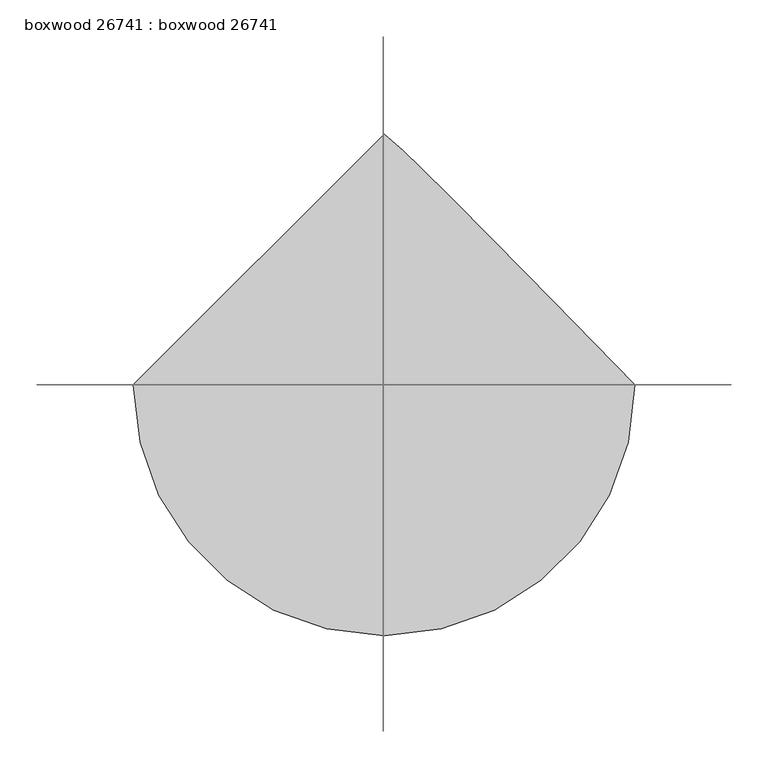
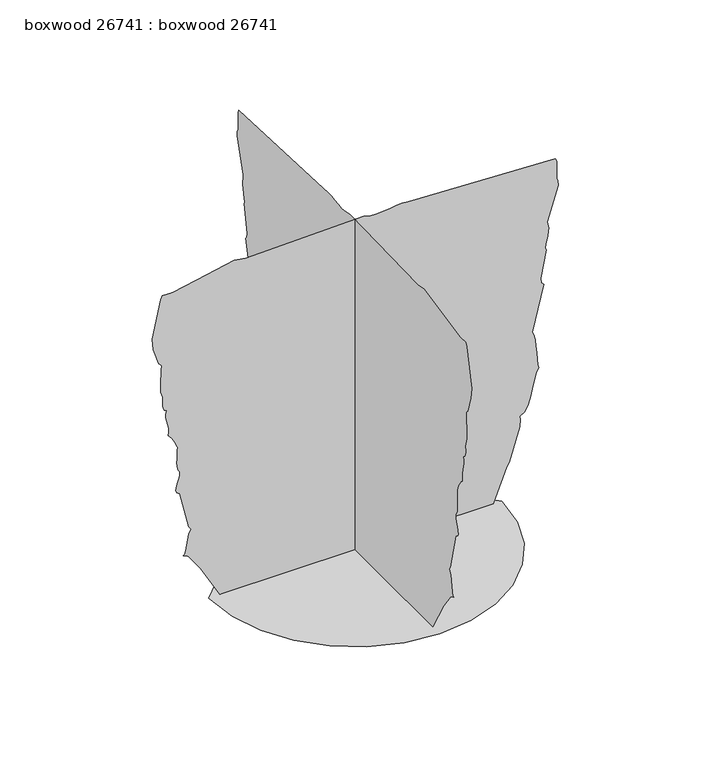
"""IFC4 building model written with IfcOpenShell, lengths in millimetres: proxy geometry, boxwood 26741 : boxwood 26741."""

from ifc_helpers import new_model, si_unit, origin, place, context, project, spatial, triangles, source, transform, mapped, element, save


def boxwood_26741_boxwood_26741_9aa5a226(model_context):
    return source(origin(), model_context, "Body", "Tessellation", [
        triangles([(-340.161904, 0.0, 0.0), (-331.1677583, -77.9424445, 0.0), (-305.5569305, -149.5201522, 0.0), (-265.3792049, -212.6823306, 0.0), (-212.6823306, -265.3792049, 0.0), (-149.5201522, -305.5569305, 0.0), (-77.9424445, -331.1677583, 0.0), (1.49e-05, -340.161904, 0.0), (77.9424445, -331.1677583, 0.0), (149.5201522, -305.5569305, 0.0), (212.6823306, -265.3792049, 0.0), (265.3792049, -212.6823306, 0.0), (305.5569305, -149.5201522, 0.0), (331.1677583, -77.9424445, 0.0), (340.161904, 2.97e-05, 0.0), (229.6165077, 113.3919522, 0.0), (147.6639246, 196.877445, 0.0), (89.5385572, 255.4401858, 0.0), (50.4748806, 294.0659713, 0.0), (25.7075946, 317.7387815, 0.0), (10.4710485, 331.4420875, 0.0), (-4.46e-05, 340.161904, 0.0), (-314.391057, 3.72e-05, 1.1804295), (-359.6030502, 3.25e-05, 80.9365932), (-387.8072153, 3.02e-05, 119.3439327), (-399.7375917, 2.98e-05, 125.1409807), (-396.5295753, 2.97e-05, 127.6759005), (-393.8092472, 2.92e-05, 136.0634881), (-391.3784363, 2.85e-05, 147.9626255), (-389.0442038, 2.77e-05, 161.0321948), (-386.6159363, 2.7e-05, 172.9315956), (-383.8930647, 2.65e-05, 181.3191832), (-380.6875917, 2.64e-05, 183.8540939), (-386.4178379, 2.59e-05, 191.475867), (-407.8706709, 2.06e-05, 279.9816748), (-415.0715758, 2.03e-05, 285.8922515), (-417.4159822, 1.99e-05, 291.1246538), (-416.3669546, 1.95e-05, 298.5846272), (-413.3773842, 1.9e-05, 307.4187355), (-409.9052124, 1.84e-05, 316.7735787), (-407.3982433, 1.79e-05, 325.7905792), (-407.3144185, 1.74e-05, 333.6213876), (-411.0989985, 1.7e-05, 339.4049735), (-412.8821019, 1.68e-05, 343.3826014), (-413.8320439, 1.64e-05, 350.1263031), (-414.1444885, 1.59e-05, 358.7927799), (-414.0123745, 1.54e-05, 368.5362259), (-413.6237718, 1.48e-05, 378.5158856), (-413.1741989, 1.42e-05, 387.8859532), (-412.8516169, 1.37e-05, 395.8056733), (-413.5475773, 1.36e-05, 397.7894185), (-415.5668581, 1.33e-05, 402.5595489), (-418.5996308, 1.29e-05, 409.0720874), (-422.335958, 1.25e-05, 416.2857096), (-426.4660111, 1.21e-05, 423.1538587), (-430.6849397, 1.17e-05, 428.6300869), (-434.6803717, 1.15e-05, 431.6729971), (-433.0471501, 1.1e-05, 440.9821309), (-433.7685087, 1.04e-05, 450.5350362), (-435.8335353, 9.9e-06, 460.1032385), (-438.2363683, 9.3e-06, 469.4580454), (-439.9737259, 8.8e-06, 478.3709098), (-440.034696, 8.3e-06, 486.6106685), (-437.4134171, 7.8e-06, 493.9512815), (-443.2020899, 7.6e-06, 497.9797056), (-446.1205164, 7.3e-06, 503.1613297), (-447.0831757, 6.9e-06, 509.2624108), (-447.0095246, 6.6e-06, 516.0543654), (-446.8114263, 6.1e-06, 523.3111536), (-447.4083012, 5.6e-06, 530.7990686), (-449.7146284, 5.2e-06, 538.2920706), (-451.312278, 4.9e-06, 544.3448625), (-452.0082384, 4.4e-06, 552.960543), (-452.0184122, 3.7e-06, 563.4380648), (-451.5713828, 3e-06, 575.0738008), (-450.8830164, 2.3e-06, 587.161653), (-450.1769185, 1.6e-06, 599.0006106), (-449.6740059, 1e-06, 609.884503), (-455.9351063, 5e-07, 616.20403), (-468.9576762, -1.9e-06, 655.9295849), (-471.3528789, -3.4e-06, 681.38806), (-452.1758881, -8.8e-06, 772.6680262), (-448.2312887, -9.3e-06, 780.8340975), (-424.9242448, -9.2e-06, 779.2695127), (-369.5370006, -9.9e-06, 791.4970367), (-280.9036933, -1.1e-05, 809.3710184), (-254.2463815, -1.07e-05, 804.8396816), (19.1367407, -1.11e-05, 811.6748022), (35.370009, -1.09e-05, 807.659059), (50.7118619, -1.08e-05, 806.6938562), (65.4184633, -1.09e-05, 807.7555647), (79.7468584, -1.1e-05, 809.8129972), (93.9523139, -1.11e-05, 811.837365), (108.2921454, -1.11e-05, 812.8000242), (123.0221057, -1.11e-05, 811.6748022), (464.7514286, -1.02e-05, 797.3212452), (467.4463586, -9.9e-06, 790.6791361), (467.5250965, -7.3e-06, 748.7767519), (470.2200628, -6.9e-06, 742.132172), (471.0074421, -6.3e-06, 730.722476), (446.1992907, -1.4e-06, 649.650753), (447.5784943, -8e-07, 638.6728621), (448.9932698, -4e-07, 632.8486536), (448.3227076, 0.0, 624.6114384), (446.3999325, 6e-07, 614.9264191), (444.0605767, 1.2e-06, 604.756255), (442.1378016, 1.8e-06, 595.0686922), (441.4672394, 2.3e-06, 586.8314406), (442.8795078, 2.7e-06, 581.0072322), (430.5681227, 6.5e-06, 516.2728114), (432.2445102, 7.2e-06, 504.59896), (437.7537669, 7.6e-06, 498.820461), (410.7154827, 1.41e-05, 389.8950966), (414.6016554, 1.45e-05, 382.811045), (417.3397877, 1.52e-05, 370.1135642), (419.2981347, 1.62e-05, 353.9591723), (420.8348505, 1.72e-05, 336.5119088), (422.3156467, 1.82e-05, 319.9231685), (424.1038007, 1.9e-05, 306.3570271), (426.5625169, 1.95e-05, 297.9699481), (420.4843268, 2.02e-05, 287.3705225), (415.6710305, 2.11e-05, 270.9595874), (411.3047636, 2.23e-05, 251.374918), (406.5625749, 2.35e-05, 231.2497293), (400.6266, 2.46e-05, 213.2215782), (392.6738514, 2.54e-05, 199.9259508), (381.8813779, 2.58e-05, 193.9993685), (383.6035111, 2.63e-05, 184.6265031), (381.7493002, 2.73e-05, 168.2889829), (357.4541988, 3.19e-05, 89.6124717), (351.8814649, 3.25e-05, 80.6919951), (319.8571115, 3.72e-05, 1.0471049), (-1.3669569, -313.0245343, 1.1804269), (-1.3669569, -358.2365275, 80.9365932), (-1.3669569, -386.4381492, 119.3439327), (-1.3669569, -398.371069, 125.1409807), (-1.3669569, -395.1630527, 127.6759005), (-1.3669569, -392.4427245, 136.0634881), (-1.3669569, -390.0119136, 147.9626255), (-1.3669569, -387.6776811, 161.0324491), (-1.3669569, -385.2469065, 172.9315956), (-1.3669569, -382.526542, 181.3191832), (-1.3669569, -379.3185256, 183.8540939), (-1.3669569, -385.0513152, 191.475867), (-1.3669569, -406.5041482, 279.9816748), (-1.3669569, -413.7050531, 285.8922515), (-1.3669569, -416.046916, 291.1246538), (-1.3669569, -414.9979248, 298.5846272), (-1.3669569, -412.0108615, 307.4187355), (-1.3669569, -408.5386897, 316.7735787), (-1.3669569, -406.0317206, 325.7905792), (-1.3669569, -405.9453524, 333.6213876), (-1.3669569, -409.7324759, 339.4049735), (-1.3669569, -411.5130358, 343.3826014), (-1.3669569, -412.4655212, 350.1263031), (-1.3669569, -412.7779658, 358.7927799), (-1.3669569, -412.6458881, 368.5362259), (-1.3669569, -412.2572491, 378.5158856), (-1.3669569, -411.8076762, 387.8859532), (-1.3669569, -411.4850942, 395.8056733), (-1.3669569, -412.1810546, 397.7894185), (-1.3669569, -414.2003354, 402.5595489), (-1.3669569, -417.2331081, 409.0720874), (-1.3669569, -420.9669282, 416.2857096), (-1.3669569, -425.0994884, 423.1538587), (-1.3669569, -429.318417, 428.6300869), (-1.3669569, -433.3113055, 431.6729971), (-1.3669569, -431.6806274, 440.9821309), (-1.3669569, -432.401986, 450.5350362), (-1.3669569, -434.4670126, 460.1032385), (-1.3669569, -436.8698456, 469.4580454), (-1.3669569, -438.6046597, 478.3709098), (-1.3669569, -438.6681733, 486.6132119), (-1.3669569, -436.0468944, 493.9512815), (-1.3669569, -441.8355672, 497.9797056), (-1.3669569, -444.75403, 503.1613297), (-1.3669569, -445.7166893, 509.2624108), (-1.3669569, -445.6430019, 516.0543654), (-1.3669569, -445.4449036, 523.3111536), (-1.3669569, -446.0417785, 530.7990686), (-1.3669569, -448.3481057, 538.2920706), (-1.3669569, -449.9457553, 544.3448625), (-1.3669569, -450.6392086, 552.960543), (-1.3669569, -450.6518895, 563.4380648), (-1.3669569, -450.2023167, 575.0738008), (-1.3669569, -449.5139866, 587.161653), (-1.3669569, -448.8078524, 599.0006106), (-1.3669569, -448.3049397, 609.884503), (-1.3669569, -454.5685836, 616.20403), (-1.3669569, -467.5911535, 655.9295849), (-1.3669569, -469.9863562, 681.38806), (-1.3669569, -450.8093654, 772.6680262), (-1.3669569, -446.864766, 780.8340975), (-1.3669569, -423.5577221, 779.2695127), (-1.3669569, -368.1704779, 791.4970367), (-1.3669569, -279.5371706, 809.3710184), (-1.3669569, -252.8793683, 804.8396816), (-1.3669569, 20.5037698, 811.6748022), (-1.3669569, 36.7367838, 807.659059), (-1.3669569, 52.0788933, 806.6938562), (-1.3669569, 66.7854902, 807.7555647), (-1.3669569, 81.1138897, 809.8129972), (-1.3669569, 95.3193453, 811.837365), (-1.3669569, 109.6591677, 812.8000242), (-1.3669569, 124.3891371, 811.6748022), (-1.3669569, 466.1179513, 797.3212452), (-1.3669569, 468.8128813, 790.6791361), (-1.3669569, 468.8916192, 748.7767519), (-1.3669569, 471.5865855, 742.132172), (-1.3669569, 472.3739648, 730.722476), (-1.3669569, 447.565777, 649.650753), (-1.3669569, 448.9475604, 638.6754055), (-1.3669569, 450.3597925, 632.8486536), (-1.3669569, 449.6892303, 624.6114384), (-1.3669569, 447.7664552, 614.9264191), (-1.3669569, 445.4270994, 604.756255), (-1.3669569, 443.5068678, 595.0686922), (-1.3669569, 442.8337621, 586.8314406), (-1.3669569, 444.2485376, 581.0072322), (-1.3669569, 431.9371888, 516.2728114), (-1.3669569, 433.6135763, 504.59896), (-1.3669569, 439.1228331, 498.820461), (-1.3669569, 412.0820054, 389.8950966), (-1.3669569, 415.9681781, 382.811045), (-1.3669569, 418.7088538, 370.1135642), (-1.3669569, 420.6646574, 353.9591723), (-1.3669569, 422.2013369, 336.5119088), (-1.3669569, 423.6821694, 319.9231685), (-1.3669569, 425.4703234, 306.3570271), (-1.3669569, 427.9290396, 297.9699481), (-1.3669569, 421.8508495, 287.3705225), (-1.3669569, 417.0375169, 270.9595874), (-1.3669569, 412.6712863, 251.374918), (-1.3669569, 407.9290976, 231.2497293), (-1.3669569, 401.9931227, 213.2215782), (-1.3669569, 394.0403741, 199.9259508), (-1.3669569, 383.2479006, 193.9993685), (-1.3669569, 384.9700338, 184.6265031), (-1.3669569, 383.1158229, 168.2892373), (-1.3669569, 358.8207215, 89.6124717), (-1.3669569, 353.2479876, 80.6919951), (-1.3669569, 321.2261776, 1.0470998)], [[21, 22, 1], [20, 21, 1], [19, 20, 1], [18, 19, 1], [17, 18, 1], [17, 1, 2], [17, 2, 3], [17, 3, 4], [16, 17, 4], [16, 4, 5], [16, 5, 6], [16, 6, 7], [16, 7, 8], [16, 8, 9], [16, 9, 10], [16, 10, 11], [16, 11, 12], [15, 16, 12], [14, 15, 12], [13, 14, 12], [25, 26, 27], [131, 132, 23], [82, 83, 84], [95, 96, 97], [95, 97, 98], [25, 27, 28], [56, 57, 58], [131, 23, 24], [130, 131, 24], [129, 130, 24], [128, 129, 24], [127, 128, 24], [95, 98, 99], [95, 99, 100], [95, 100, 101], [95, 101, 102], [127, 24, 25], [127, 25, 28], [127, 28, 29], [127, 29, 30], [127, 30, 31], [127, 31, 32], [127, 32, 33], [127, 33, 34], [127, 34, 35], [111, 112, 113], [95, 102, 103], [95, 103, 104], [95, 104, 105], [95, 105, 106], [95, 106, 107], [95, 107, 108], [119, 120, 121], [81, 82, 84], [95, 108, 109], [95, 109, 110], [94, 95, 110], [93, 94, 110], [92, 93, 110], [91, 92, 110], [91, 110, 111], [90, 91, 111], [90, 111, 113], [89, 90, 113], [126, 127, 35], [125, 126, 35], [124, 125, 35], [123, 124, 35], [122, 123, 35], [121, 122, 35], [119, 121, 35], [118, 119, 35], [117, 118, 35], [116, 117, 35], [115, 116, 35], [114, 115, 35], [113, 114, 35], [89, 113, 35], [88, 89, 35], [87, 88, 35], [87, 35, 36], [87, 36, 37], [81, 84, 85], [80, 81, 85], [79, 80, 85], [78, 79, 85], [78, 85, 86], [78, 86, 87], [77, 78, 87], [76, 77, 87], [75, 76, 87], [74, 75, 87], [73, 74, 87], [72, 73, 87], [71, 72, 87], [70, 71, 87], [69, 70, 87], [68, 69, 87], [67, 68, 87], [66, 67, 87], [65, 66, 87], [64, 65, 87], [55, 56, 58], [62, 63, 64], [62, 64, 87], [61, 62, 87], [60, 61, 87], [59, 60, 87], [58, 59, 87], [55, 58, 87], [54, 55, 87], [53, 54, 87], [52, 53, 87], [51, 52, 87], [50, 51, 87], [49, 50, 87], [48, 49, 87], [47, 48, 87], [46, 47, 87], [45, 46, 87], [44, 45, 87], [43, 44, 87], [42, 43, 87], [41, 42, 87], [37, 38, 39], [37, 39, 40], [87, 37, 40], [41, 87, 40], [135, 136, 137], [241, 242, 133], [192, 193, 194], [205, 206, 207], [205, 207, 208], [135, 137, 138], [166, 167, 168], [241, 133, 134], [240, 241, 134], [239, 240, 134], [238, 239, 134], [237, 238, 134], [205, 208, 209], [205, 209, 210], [205, 210, 211], [205, 211, 212], [237, 134, 135], [237, 135, 138], [237, 138, 139], [237, 139, 140], [237, 140, 141], [237, 141, 142], [237, 142, 143], [237, 143, 144], [237, 144, 145], [221, 222, 223], [205, 212, 213], [205, 213, 214], [205, 214, 215], [205, 215, 216], [205, 216, 217], [205, 217, 218], [229, 230, 231], [191, 192, 194], [205, 218, 219], [205, 219, 220], [204, 205, 220], [203, 204, 220], [202, 203, 220], [201, 202, 220], [201, 220, 221], [200, 201, 221], [200, 221, 223], [199, 200, 223], [236, 237, 145], [235, 236, 145], [234, 235, 145], [233, 234, 145], [232, 233, 145], [231, 232, 145], [229, 231, 145], [228, 229, 145], [227, 228, 145], [226, 227, 145], [225, 226, 145], [224, 225, 145], [223, 224, 145], [199, 223, 145], [198, 199, 145], [197, 198, 145], [197, 145, 146], [197, 146, 147], [191, 194, 195], [190, 191, 195], [189, 190, 195], [188, 189, 195], [188, 195, 196], [188, 196, 197], [187, 188, 197], [186, 187, 197], [185, 186, 197], [184, 185, 197], [183, 184, 197], [182, 183, 197], [181, 182, 197], [180, 181, 197], [179, 180, 197], [178, 179, 197], [177, 178, 197], [176, 177, 197], [175, 176, 197], [174, 175, 197], [165, 166, 168], [172, 173, 174], [172, 174, 197], [171, 172, 197], [170, 171, 197], [169, 170, 197], [168, 169, 197], [165, 168, 197], [164, 165, 197], [163, 164, 197], [162, 163, 197], [161, 162, 197], [160, 161, 197], [159, 160, 197], [158, 159, 197], [157, 158, 197], [156, 157, 197], [155, 156, 197], [154, 155, 197], [153, 154, 197], [152, 153, 197], [151, 152, 197], [147, 148, 149], [147, 149, 150], [197, 147, 150], [151, 197, 150]], closed=False),
    ])


if __name__ == "__main__":
    model = new_model("IFC4")
    model_context = context("Model", 3, world=origin())
    ifc_project = project(units=[si_unit("LENGTHUNIT", "METRE", prefix="MILLI")], contexts=[model_context])
    site = spatial("IfcSite", under=ifc_project)
    building = spatial("IfcBuilding", under=site)
    placement = place(None, origin())
    boxwood_26741_boxwood_26741_shape = boxwood_26741_boxwood_26741_9aa5a226(model_context)
    element("IfcBuildingElementProxy", 1, Name="boxwood 26741 : boxwood 26741", ObjectType="boxwood 26741 : boxwood 26741", at=placement, inside=building, context=model_context, shape_type="MappedRepresentation", body=[
        mapped(boxwood_26741_boxwood_26741_shape, transform((0.0, 0.0, 0.0), x_axis=(1.0, 0.0, 0.0), y_axis=(0.0, 1.0, 0.0), z_axis=(0.0, 0.0, 1.0))),
    ])
    save(model, "model.ifc")

# Revit data of these elements
# Type "boxwood 26741 : boxwood 26741"
#   built-in parameter 1005195 = "RPC-16-G0M3-8AG0-UBW3-U000-ST1L-LVER-AU"
#   Height = 0
